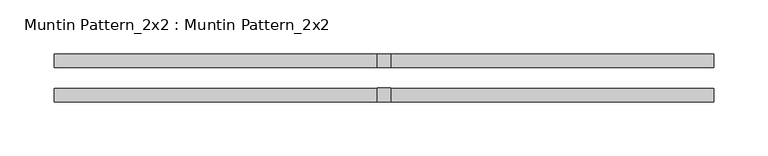
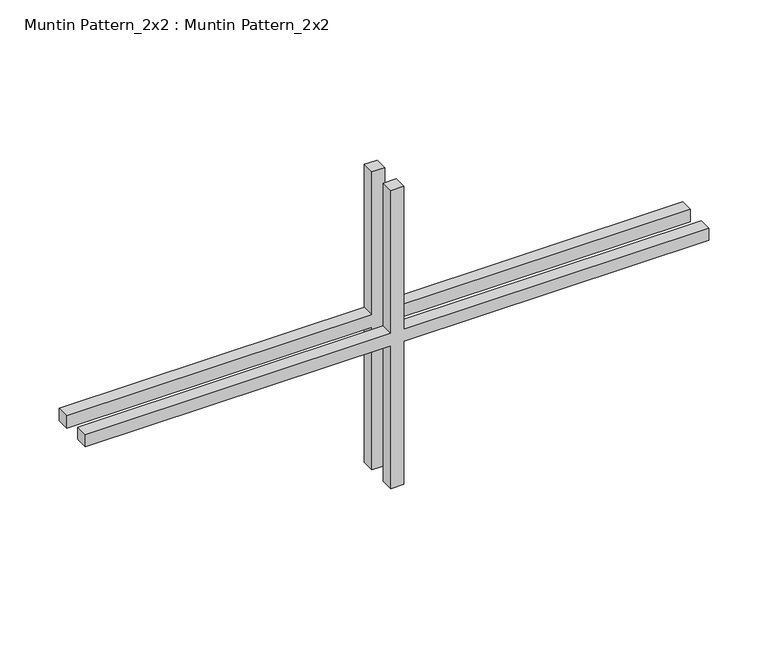
"""IFC4 building model written with IfcOpenShell, lengths in millimetres: proxy geometry, Muntin Pattern_2x2 : Muntin Pattern_2x2."""

import ifcopenshell
import ifcopenshell.guid

model = None  # the IFC model being written
_history = None  # IfcOwnerHistory: only IFC2X3 demands one
_inside = {}  # id of a spatial element -> (the spatial element, [elements in it])
_under = {}  # id of a project, library or spatial element -> (it, [spatial elements below it])
_declared = {}  # id of a project -> (the project, [libraries it declares])
_typed = {}  # id of a type object -> (the type object, [elements of that type])
_made_of = {}  # id of a material, layer set ... -> (it, [elements and type objects made of it])


def new_model(schema):
    """Start an empty IFC model of exactly this schema.

    Asked for "IFC4X3", IfcOpenShell would pick the latest addendum, in which some entities
    have other attributes; the version numbers below select the first issue.
    IFC2X3 requires an IfcOwnerHistory on every rooted entity: one is made here for all.
    """
    global model, _history
    if schema == "IFC4X3":
        model = ifcopenshell.file(schema_version=(4, 3, 0, 0))
    else:
        model = ifcopenshell.file(schema=schema)
    _inside.clear()
    _under.clear()
    _declared.clear()
    _typed.clear()
    _made_of.clear()
    _history = None
    if model.schema == "IFC2X3":
        org = make("IfcOrganization", Name="unknown")
        user = make(
            "IfcPersonAndOrganization",
            ThePerson=make("IfcPerson", FamilyName="unknown"),
            TheOrganization=org,
        )
        app = make(
            "IfcApplication",
            ApplicationDeveloper=org,
            Version="unknown",
            ApplicationFullName="unknown",
            ApplicationIdentifier="unknown",
        )
        _history = make(
            "IfcOwnerHistory",
            OwningUser=user,
            OwningApplication=app,
            ChangeAction="ADDED",
            CreationDate=0,
        )
    return model


def make(cls, **values):
    """One entity of the class cls with the attributes given. An attribute that is None is left unset."""
    return model.create_entity(
        cls, **{name: value for name, value in values.items() if value is not None}
    )


def rooted(cls, **values):
    """An entity with a GlobalId (a new one), such as an element, a storey or a relation."""
    return make(cls, GlobalId=ifcopenshell.guid.new(), OwnerHistory=_history, **values)


def si_unit(unit_type, name, prefix=None):
    """IfcSIUnit, for example si_unit("LENGTHUNIT", "METRE", prefix="MILLI")."""
    return make("IfcSIUnit", UnitType=unit_type, Prefix=prefix, Name=name)


def assignment(units):
    """IfcUnitAssignment: the units of a project."""
    return None if units is None else make("IfcUnitAssignment", Units=units)


def point(xyz):
    """IfcCartesianPoint."""
    return None if xyz is None else make("IfcCartesianPoint", Coordinates=xyz)


def direction(xyz):
    """IfcDirection."""
    return None if xyz is None else make("IfcDirection", DirectionRatios=xyz)


def frame(location, z_axis=None, x_axis=None):
    """IfcAxis2Placement3D, a coordinate frame: its origin and axes. An axis left out is left unset."""
    return make(
        "IfcAxis2Placement3D",
        Location=point(location),
        Axis=direction(z_axis),
        RefDirection=direction(x_axis),
    )


def origin():
    """The frame at (0, 0, 0) with its axes left unset."""
    return frame((0.0, 0.0, 0.0))


def place(relative_to, where):
    """IfcLocalPlacement: puts the frame where relative to a parent placement (None: the world)."""
    return make(
        "IfcLocalPlacement", PlacementRelTo=relative_to, RelativePlacement=where
    )


def context(
    kind, dimensions, precision=None, world=None, true_north=None, identifier=None
):
    """IfcGeometricRepresentationContext, for example the 3D "Model" context."""
    return make(
        "IfcGeometricRepresentationContext",
        ContextIdentifier=identifier,
        ContextType=kind,
        CoordinateSpaceDimension=dimensions,
        Precision=precision,
        WorldCoordinateSystem=world,
        TrueNorth=true_north,
    )


def project(units=None, contexts=None):
    """IfcProject with its units and contexts."""
    return rooted(
        "IfcProject",
        Name="project",
        RepresentationContexts=contexts,
        UnitsInContext=assignment(units),
    )


def spatial(cls, under=None, at=None, **own):
    """A site, building, storey or space (cls), placed at a placement, below another one or the project."""
    s = rooted(cls, ObjectPlacement=at, **own)
    if under is not None:
        _under.setdefault(under.id(), (under, []))[1].append(s)
    return s


def polyline(points):
    """IfcPolyline through the points."""
    return make("IfcPolyline", Points=[point(p) for p in points])


def outline(outer, holes=None, kind="AREA"):
    """IfcArbitraryClosedProfileDef: a profile drawn as a closed curve; with holes, ...WithVoids."""
    if holes is None:
        return make("IfcArbitraryClosedProfileDef", ProfileType=kind, OuterCurve=outer)
    return make(
        "IfcArbitraryProfileDefWithVoids",
        ProfileType=kind,
        OuterCurve=outer,
        InnerCurves=holes,
    )


def extrude(swept, where, along, depth):
    """IfcExtrudedAreaSolid: the profile swept, set in the frame where, extruded along a direction by depth."""
    return make(
        "IfcExtrudedAreaSolid",
        SweptArea=swept,
        Position=where,
        ExtrudedDirection=direction(along),
        Depth=depth,
    )


def shape(context_of_items, identifier, shape_type, items):
    """IfcShapeRepresentation: the items that make up one representation, for example the "Body"."""
    return make(
        "IfcShapeRepresentation",
        ContextOfItems=context_of_items,
        RepresentationIdentifier=identifier,
        RepresentationType=shape_type,
        Items=items,
    )


def source(mapping_origin, context_of_items, identifier, shape_type, items):
    """IfcRepresentationMap: a shape defined once, which mapped items show again and again."""
    return make(
        "IfcRepresentationMap",
        MappingOrigin=mapping_origin,
        MappedRepresentation=shape(context_of_items, identifier, shape_type, items),
    )


def transform(
    local_origin,
    x_axis=None,
    y_axis=None,
    z_axis=None,
    scale=None,
    scale2=None,
    scale3=None,
    uniform=True,
):
    """IfcCartesianTransformationOperator3D, or its non-uniform kind. x_axis, y_axis, z_axis: its Axis1, 2, 3."""
    if uniform:
        return make(
            "IfcCartesianTransformationOperator3D",
            Axis1=direction(x_axis),
            Axis2=direction(y_axis),
            LocalOrigin=point(local_origin),
            Scale=scale,
            Axis3=direction(z_axis),
        )
    return make(
        "IfcCartesianTransformationOperator3DnonUniform",
        Axis1=direction(x_axis),
        Axis2=direction(y_axis),
        LocalOrigin=point(local_origin),
        Scale=scale,
        Axis3=direction(z_axis),
        Scale2=scale2,
        Scale3=scale3,
    )


def mapped(mapping_source, mapping_target):
    """IfcMappedItem: shows the shape of a source again, moved by a transform."""
    return make(
        "IfcMappedItem", MappingSource=mapping_source, MappingTarget=mapping_target
    )


def made_of(thing, what):
    """Note that an element or type object is made of a material, layer set ...; save() writes the relation."""
    if what is not None:
        _made_of.setdefault(what.id(), (what, []))[1].append(thing)
    return thing


def element(
    cls,
    number,
    at=None,
    inside=None,
    cuts=None,
    type_object=None,
    material=None,
    context=None,
    identifier="Body",
    shape_type=None,
    held_by="IfcProductDefinitionShape",
    body=None,
    shapes=None,
    **own,
):
    """One element of the class cls, such as IfcWall. Its Tag is "e" and its number.

    at: its placement. inside: the storey or other place that contains it. cuts: it is an
    opening in that element (IfcRelVoidsElement). A single representation is given by context,
    identifier, shape_type and body (its items); several are given by shapes. held_by: the class
    of the entity that holds the representations. save() writes the other relations.
    """
    e = rooted(cls, Tag="e%d" % number, ObjectPlacement=at, **own)
    if body is not None:
        shapes = [shape(context, identifier, shape_type, body)]
    if shapes is not None:
        e.Representation = make(held_by, Representations=shapes)
    if inside is not None:
        _inside.setdefault(inside.id(), (inside, []))[1].append(e)
    if cuts is not None:
        rooted(
            "IfcRelVoidsElement", RelatingBuildingElement=cuts, RelatedOpeningElement=e
        )
    if type_object is not None:
        _typed.setdefault(type_object.id(), (type_object, []))[1].append(e)
    return made_of(e, material)


def aggregate(whole, parts):
    """IfcRelAggregates: a whole, such as a stair, and the parts it consists of."""
    return rooted("IfcRelAggregates", RelatingObject=whole, RelatedObjects=parts)


def save(model, path):
    """Write the relations noted so far, then the file.

    IfcRelAggregates (storeys below a building ...), IfcRelContainedInSpatialStructure (elements
    in a storey), IfcRelDefinesByType, IfcRelAssociatesMaterial and IfcRelDeclares: one each for
    every whole, place, type object, material and project.
    """
    for whole, parts in _under.values():
        aggregate(whole, parts)
    for where, things in _inside.values():
        rooted(
            "IfcRelContainedInSpatialStructure",
            RelatedElements=things,
            RelatingStructure=where,
        )
    for kind, things in _typed.values():
        rooted("IfcRelDefinesByType", RelatedObjects=things, RelatingType=kind)
    for what, things in _made_of.values():
        rooted("IfcRelAssociatesMaterial", RelatedObjects=things, RelatingMaterial=what)
    for by, libraries in _declared.values():
        rooted("IfcRelDeclares", RelatingContext=by, RelatedDefinitions=libraries)
    model.write(path)


def muntin_pattern_2x2_muntin_pattern_2x2_a77e86ff(model_context):
    return source(origin(), model_context, "Body", "SweptSolid", [
        extrude(outline(polyline([(160.3375, -6.35), (160.3375, -304.8), (147.6375, -304.8), (147.6375, -6.35), (0.0, -6.35), (0.0, 6.35), (147.6375, 6.35), (147.6375, 304.8), (160.3375, 304.8), (160.3375, 6.35), (307.975, 6.35), (307.975, -6.35), (160.3375, -6.35)])), frame((0.0, 9.525, 0.0), z_axis=(0.0, 1.0, 0.0), x_axis=(0.0, 0.0, 1.0)), (0.0, 0.0, 1.0), 12.7),
        extrude(outline(polyline([(160.3375, -6.35), (160.3375, -304.8), (147.6375, -304.8), (147.6375, -6.35), (0.0, -6.35), (0.0, 6.35), (147.6375, 6.35), (147.6375, 304.8), (160.3375, 304.8), (160.3375, 6.35), (307.975, 6.35), (307.975, -6.35), (160.3375, -6.35)])), frame((0.0, -22.225, 0.0), z_axis=(0.0, 1.0, 0.0), x_axis=(0.0, 0.0, 1.0)), (0.0, 0.0, 1.0), 12.7),
    ])


if __name__ == "__main__":
    model = new_model("IFC4")
    model_context = context("Model", 3, world=origin())
    ifc_project = project(units=[si_unit("LENGTHUNIT", "METRE", prefix="MILLI")], contexts=[model_context])
    site = spatial("IfcSite", under=ifc_project)
    building = spatial("IfcBuilding", under=site)
    placement = place(None, origin())
    muntin_pattern_2x2_muntin_pattern_2x2_shape = muntin_pattern_2x2_muntin_pattern_2x2_a77e86ff(model_context)
    element("IfcBuildingElementProxy", 1, Name="Muntin Pattern_2x2 : Muntin Pattern_2x2", ObjectType="Muntin Pattern_2x2 : Muntin Pattern_2x2", at=placement, inside=building, context=model_context, shape_type="MappedRepresentation", body=[
        mapped(muntin_pattern_2x2_muntin_pattern_2x2_shape, transform((0.0, 0.0, 0.0), x_axis=(1.0, 0.0, 0.0), y_axis=(0.0, 1.0, 0.0), z_axis=(0.0, 0.0, 1.0))),
    ])
    save(model, "model.ifc")

# Revit data of these elements
# Type "Muntin Pattern_2x2 : Muntin Pattern_2x2"
#   Width [instance default] = 4' - 0"
#   Thickness = 0' - 0 1/2"
#   Height [instance default] = 4' - 0"
#   Distance = 0' - 0 3/4"
#   Interior Material [instance default] = none
#   Exterior Material [instance default] = none
# Element 1 (IfcBuildingElementProxy, "Muntin Pattern_2x2 : Muntin Pattern_2x2")
#   Width = 2' - 0"
#   Height = 1' - 0 1/8"
#   Interior Material = Wood - Stained
#   Exterior Material = Clad - White
#   Materials on its faces: "Clad - White", "Wood - Stained"
# Materials
#   "Clad - White": class "Wood", colour RGB 242 242 238, transparency 0, Cost = 0
#   "Wood - Stained": class "Wood", colour RGB 224 178 126, transparency 0, Cost = 0
